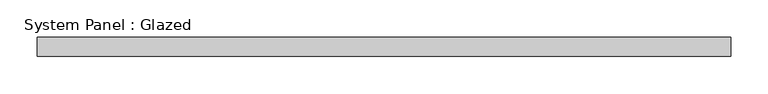
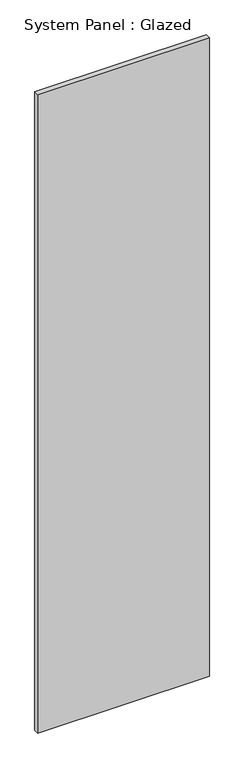
"""IFC4 building model written with IfcOpenShell, lengths in millimetres: plate geometry, System Panel : Glazed."""

from ifc_helpers import new_model, si_unit, origin, origin_with_axes, place, context, project, spatial, polyline, outline, extrude, source, transform, mapped, element, save


def system_panel_glazed_b062bbc2(model_context):
    return source(origin(), model_context, "Body", "SweptSolid", [
        extrude(outline(polyline([(465.8483058, -44.45), (-465.8483058, -44.45), (-465.8483058, -19.05), (465.8483058, -19.05), (465.8483058, -44.45)])), origin_with_axes(), (0.0, 0.0, 1.0), 3657.6),
    ])


if __name__ == "__main__":
    model = new_model("IFC4")
    model_context = context("Model", 3, world=origin())
    ifc_project = project(units=[si_unit("LENGTHUNIT", "METRE", prefix="MILLI")], contexts=[model_context])
    site = spatial("IfcSite", under=ifc_project)
    building = spatial("IfcBuilding", under=site)
    placement = place(None, origin())
    system_panel_glazed_shape = system_panel_glazed_b062bbc2(model_context)
    element("IfcPlate", 1, ObjectType="System Panel : Glazed", at=placement, inside=building, context=model_context, shape_type="MappedRepresentation", body=[
        mapped(system_panel_glazed_shape, transform((0.0, 0.0, 0.0), x_axis=(1.0, 0.0, 0.0), y_axis=(0.0, 1.0, 0.0), z_axis=(0.0, 0.0, 1.0))),
    ])
    save(model, "model.ifc")

# Revit data of these elements
# Type "System Panel : Glazed"
#   Construction Type Id = "GSP4R"
#   Analytic Construction = "1/8 in Pilkington single glazing"
#   Visual Light Transmittance = 0.9
#   Solar Heat Gain Coefficient = 0.86
#   Heat Transfer Coefficient (U) = 1.18115 BTU/(h·ft²·°F)
#   Define Thermal Properties by = 1
# Element 1 (IfcPlate, "System Panel : Glazed")
#   Materials on its faces: "Glass"
# Materials
#   "Glass": class "Glass", colour RGB 0 128 192, transparency 0.75, Description = "Soda Lime Glass", Cost = 0
